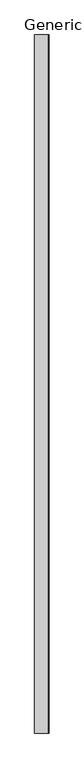
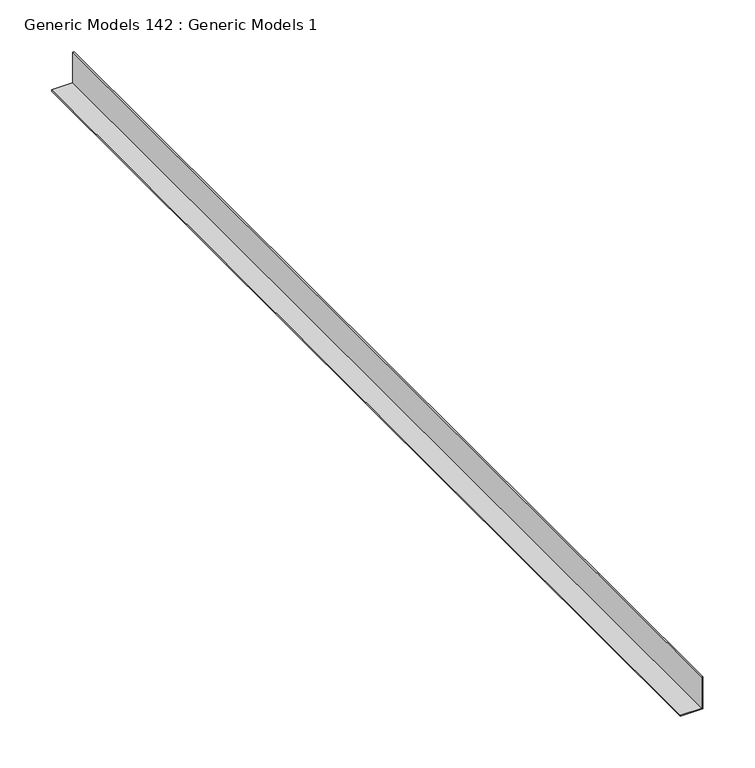
"""IFC4 building model written with IfcOpenShell, lengths in millimetres: proxy geometry, Generic Models 142 : Generic Models 1."""

from ifc_helpers import new_model, si_unit, frame, origin, place, context, project, spatial, polyline, outline, extrude, source, transform, mapped, element, save


def generic_models_142_generic_models_1_b1789cf9(model_context):
    return source(origin(), model_context, "Body", "SweptSolid", [
        extrude(outline(polyline([(126.6971102, 49694.3681639), (126.6971102, 49692.7806639), (90.1846102, 49692.7806639), (90.1846102, 49668.9681639), (88.5971102, 49668.9681639), (88.5971102, 49694.3681639), (126.6971102, 49694.3681639)])), frame((0.0, 0.0, 0.0), z_axis=(0.0, 1.0, 0.0), x_axis=(0.0, 0.0, 1.0)), (0.0, 0.0, 1.0), 1219.2),
    ])


if __name__ == "__main__":
    model = new_model("IFC4")
    model_context = context("Model", 3, world=origin())
    ifc_project = project(units=[si_unit("LENGTHUNIT", "METRE", prefix="MILLI")], contexts=[model_context])
    site = spatial("IfcSite", under=ifc_project)
    building = spatial("IfcBuilding", under=site)
    placement = place(None, origin())
    generic_models_142_generic_models_1_shape = generic_models_142_generic_models_1_b1789cf9(model_context)
    element("IfcBuildingElementProxy", 1, Name="Generic Models 142 : Generic Models 1", ObjectType="Generic Models 142 : Generic Models 1", at=placement, inside=building, context=model_context, shape_type="MappedRepresentation", body=[
        mapped(generic_models_142_generic_models_1_shape, transform((0.0, 0.0, 0.0), x_axis=(1.0, 0.0, 0.0), y_axis=(0.0, 1.0, 0.0), z_axis=(0.0, 0.0, 1.0))),
    ])
    save(model, "model.ifc")

# Revit data of these elements
# Element 1 (IfcBuildingElementProxy, "Generic Models 142 : Generic Models 1")
#   Materials on its faces: "CEILING TRACK TO MATCH EXISTING"
# Materials
#   "CEILING TRACK TO MATCH EXISTING": class "Unassigned", colour RGB 210 209 208, transparency 0, Keynote = "M05121300.02", Cost = 0
